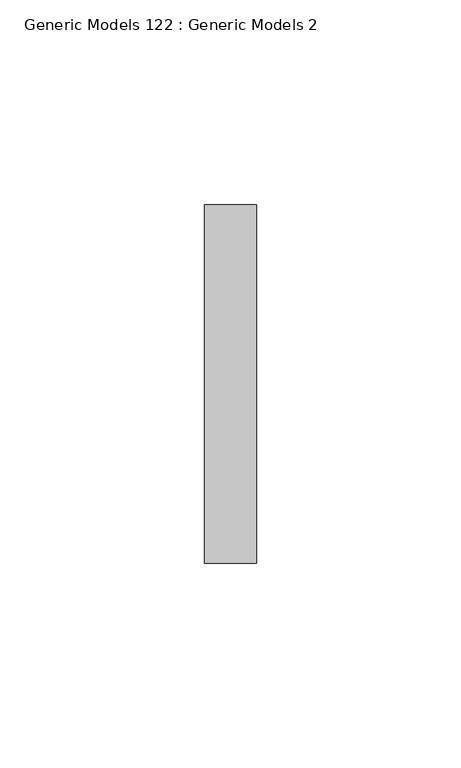
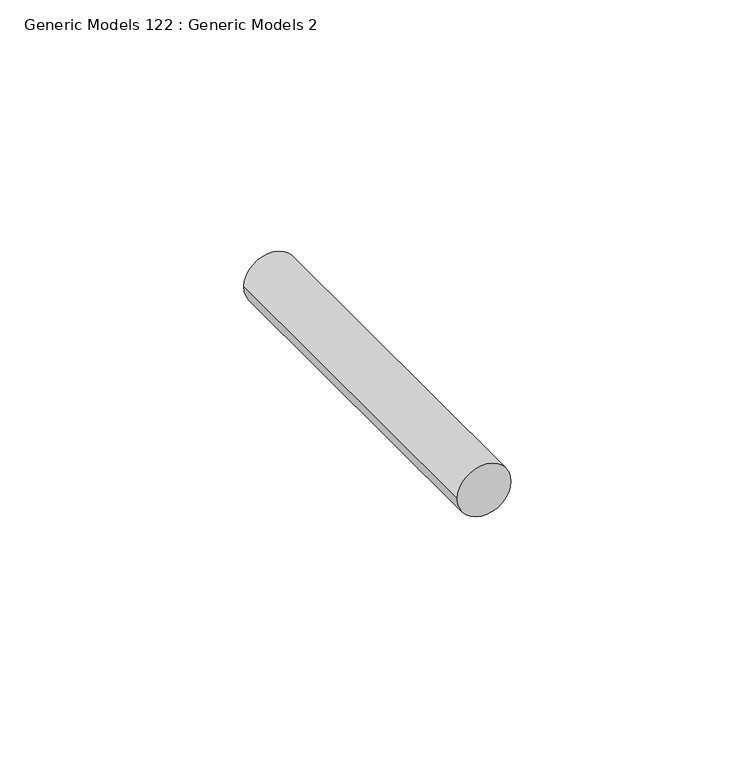
"""IFC4 building model written with IfcOpenShell, lengths in millimetres: proxy geometry, Generic Models 122 : Generic Models 2."""

from ifc_helpers import new_model, si_unit, point, frame, frame_2d, origin, place, context, project, spatial, circle_curve, trimmed, segment, composite_curve, outline, extrude, source, transform, mapped, element, save


def generic_models_122_generic_models_2_80e3af58(model_context):
    return source(origin(), model_context, "Body", "SweptSolid", [
        extrude(outline(composite_curve([segment(trimmed(circle_curve(frame_2d((38203.4419837, 7407.5828124)), 6.35), [point((38203.4419837, 7401.2328124))], [point((38203.4419837, 7413.9328124))], False, "CARTESIAN"), True, "CONTINUOUS"), segment(trimmed(circle_curve(frame_2d((38203.4419837, 7407.5828124)), 6.35), [point((38203.4419837, 7413.9328124))], [point((38203.4419837, 7401.2328124))], False, "CARTESIAN"), True, "CONTINUOUS")], self_intersect=False)), frame((0.0, 1848.3666731, 0.0), z_axis=(0.0, 1.0, 0.0), x_axis=(0.0, 0.0, 1.0)), (0.0, 0.0, 1.0), 87.551022),
    ])


if __name__ == "__main__":
    model = new_model("IFC4")
    model_context = context("Model", 3, world=origin())
    ifc_project = project(units=[si_unit("LENGTHUNIT", "METRE", prefix="MILLI")], contexts=[model_context])
    site = spatial("IfcSite", under=ifc_project)
    building = spatial("IfcBuilding", under=site)
    placement = place(None, origin())
    generic_models_122_generic_models_2_shape = generic_models_122_generic_models_2_80e3af58(model_context)
    element("IfcBuildingElementProxy", 1, Name="Generic Models 122 : Generic Models 2", ObjectType="Generic Models 122 : Generic Models 2", at=placement, inside=building, context=model_context, shape_type="MappedRepresentation", body=[
        mapped(generic_models_122_generic_models_2_shape, transform((0.0, 0.0, 0.0), x_axis=(1.0, 0.0, 0.0), y_axis=(0.0, 1.0, 0.0), z_axis=(0.0, 0.0, 1.0))),
    ])
    save(model, "model.ifc")

# Revit data of these elements
# Element 1 (IfcBuildingElementProxy, "Generic Models 122 : Generic Models 2")
#   Materials on its faces: "S.S. LAG BOLT - SEE STRUCT. DWGS"
# Materials
#   "S.S. LAG BOLT - SEE STRUCT. DWGS": class "Generic", colour RGB 120 120 120, transparency 0, Cost = 0
